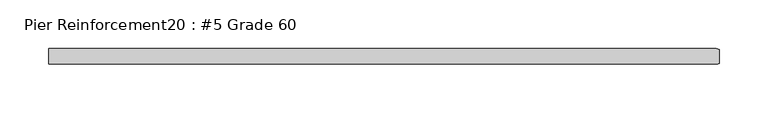
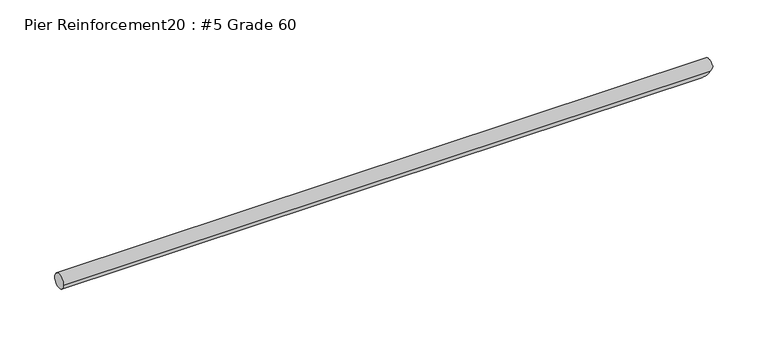
"""IFC4 building model written with IfcOpenShell, lengths in millimetres: proxy geometry, Pier Reinforcement20 : #5 Grade 60."""

from ifc_helpers import new_model, si_unit, frame, origin, place, context, project, spatial, circle_curve, ellipse_curve, source, transform, mapped, element, save
from ifc_brep_helpers import plane_surface, cylinder_surface, advanced_brep


def pier_reinforcement20_5_grade_60_3385e020(model_context):
    return source(origin(), model_context, "Body", "AdvancedBrep", [
        advanced_brep(
        [(590233.9922365, -534089.3915452, -52.3875), (590233.9922365, -534103.941223, -52.3875), (589548.1922365, -534088.7288841, -55.5625), (589548.1922365, -534104.6038841, -55.5625), (590230.8172365, -534104.6038841, -55.5625), (590230.8172365, -534088.7288841, -55.5625), (590222.8797365, -534096.6663841, -63.5)],
        [
            (0, 1, circle_curve(frame((590233.9922365, -534096.6663841, -55.5625), z_axis=(1.0, 0.0, 0.0), x_axis=(0.0, -1.0, 0.0)), 7.9375)),
            (1, 0),
            (2, 3, circle_curve(frame((589548.1922365, -534096.6663841, -55.5625), z_axis=(-1.0, 0.0, 0.0), x_axis=(0.0, -1.0, 0.0)), 7.9375)),
            (3, 2, circle_curve(frame((589548.1922365, -534096.6663841, -55.5625), z_axis=(-1.0, 0.0, 0.0), x_axis=(0.0, -1.0, 0.0)), 7.9375)),
            (3, 4),
            (4, 1, ellipse_curve(frame((590230.8172365, -534096.6663841, -55.5625), z_axis=(-0.7071067811865462, 0.0, 0.7071067811865489), x_axis=(0.7071067811865487, 0.0, 0.7071067811865462)), 11.2253202, 7.9375)),
            (0, 5, ellipse_curve(frame((590230.8172365, -534096.6663841, -55.5625), z_axis=(-0.7071067811865462, 0.0, 0.7071067811865489), x_axis=(0.7071067811865487, 0.0, 0.7071067811865462)), 11.2253202, 7.9375)),
            (5, 2),
            (5, 6, ellipse_curve(frame((590230.8172365, -534096.6663841, -55.5625), z_axis=(-0.7071067811865462, 0.0, 0.7071067811865489), x_axis=(0.7071067811865487, 0.0, 0.7071067811865462)), 11.2253202, 7.9375)),
            (6, 4, ellipse_curve(frame((590230.8172365, -534096.6663841, -55.5625), z_axis=(-0.7071067811865462, 0.0, 0.7071067811865489), x_axis=(0.7071067811865487, 0.0, 0.7071067811865462)), 11.2253202, 7.9375)),
        ],
        [
            plane_surface(frame((590233.9922365, -534104.6038841, -55.5625), z_axis=(1.0, 0.0, 0.0), x_axis=(0.0, 0.0, -1.0))),
            plane_surface(frame((589548.1922365, -534104.6038841, -55.5625), z_axis=(-1.0, 0.0, 0.0), x_axis=(0.0, 0.0, 1.0))),
            cylinder_surface(frame((589548.1922365, -534096.6663841, -55.5625), z_axis=(1.0, 0.0, 0.0), x_axis=(0.0, -1.0, 0.0)), 7.9375),
            plane_surface(frame((590222.8797365, -534128.4163841, -63.5), z_axis=(0.7071067811865462, 0.0, -0.7071067811865489), x_axis=(0.0, 1.0, 0.0))),
        ],
        [
            (0, [[1, 2]]),
            (1, [[3, 4]]),
            (2, [[-4, 5, 6, -1, 7, 8]]),
            (2, [[-3, -8, 9, 10, -5]]),
            (3, [[-2, -6, -10, -9, -7]]),
        ],
    ),
    ])


if __name__ == "__main__":
    model = new_model("IFC4")
    model_context = context("Model", 3, world=origin())
    ifc_project = project(units=[si_unit("LENGTHUNIT", "METRE", prefix="MILLI")], contexts=[model_context])
    site = spatial("IfcSite", under=ifc_project)
    building = spatial("IfcBuilding", under=site)
    placement = place(None, origin())
    pier_reinforcement20_5_grade_60_shape = pier_reinforcement20_5_grade_60_3385e020(model_context)
    element("IfcBuildingElementProxy", 1, Name="Pier Reinforcement20 : #5 Grade 60", ObjectType="Pier Reinforcement20 : #5 Grade 60", at=placement, inside=building, context=model_context, shape_type="MappedRepresentation", body=[
        mapped(pier_reinforcement20_5_grade_60_shape, transform((0.0, 0.0, 0.0), x_axis=(1.0, 0.0, 0.0), y_axis=(0.0, 1.0, 0.0), z_axis=(0.0, 0.0, 1.0))),
    ])
    save(model, "model.ifc")

# Revit data of these elements
# Element 1 (IfcBuildingElementProxy, "Pier Reinforcement20 : #5 Grade 60")
#   Materials on its faces: "#4 GR. 60 REINF. @ 16\" O.C. EW."
# Materials
#   "#4 GR. 60 REINF. @ 16\" O.C. EW.": class "Generic", colour RGB 84 83 81, transparency 0, Cost = 0
